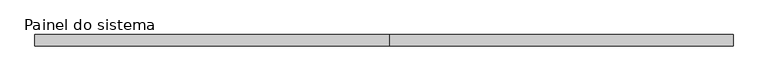
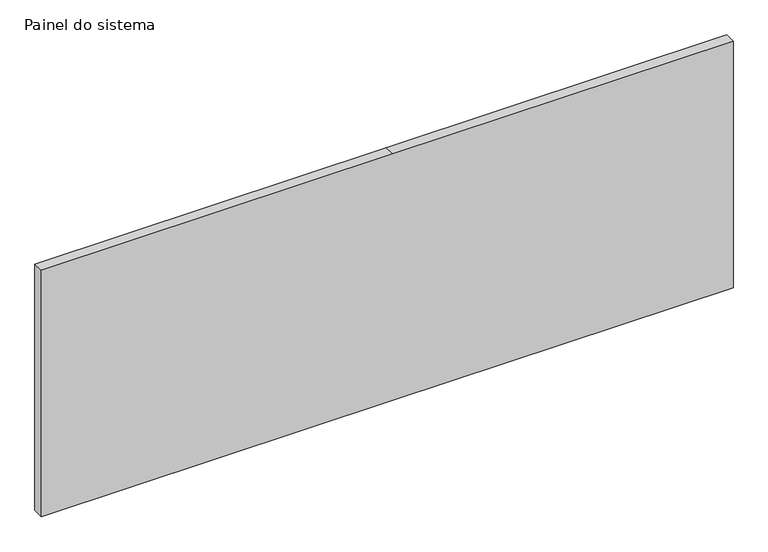
"""IFC4 building model written with IfcOpenShell, lengths in millimetres: plate geometry, Painel do sistema : Envidraçado."""

import ifcopenshell
import ifcopenshell.guid

model = None  # the IFC model being written
_history = None  # IfcOwnerHistory: only IFC2X3 demands one
_inside = {}  # id of a spatial element -> (the spatial element, [elements in it])
_under = {}  # id of a project, library or spatial element -> (it, [spatial elements below it])
_declared = {}  # id of a project -> (the project, [libraries it declares])
_typed = {}  # id of a type object -> (the type object, [elements of that type])
_made_of = {}  # id of a material, layer set ... -> (it, [elements and type objects made of it])


def new_model(schema):
    """Start an empty IFC model of exactly this schema.

    Asked for "IFC4X3", IfcOpenShell would pick the latest addendum, in which some entities
    have other attributes; the version numbers below select the first issue.
    IFC2X3 requires an IfcOwnerHistory on every rooted entity: one is made here for all.
    """
    global model, _history
    if schema == "IFC4X3":
        model = ifcopenshell.file(schema_version=(4, 3, 0, 0))
    else:
        model = ifcopenshell.file(schema=schema)
    _inside.clear()
    _under.clear()
    _declared.clear()
    _typed.clear()
    _made_of.clear()
    _history = None
    if model.schema == "IFC2X3":
        org = make("IfcOrganization", Name="unknown")
        user = make(
            "IfcPersonAndOrganization",
            ThePerson=make("IfcPerson", FamilyName="unknown"),
            TheOrganization=org,
        )
        app = make(
            "IfcApplication",
            ApplicationDeveloper=org,
            Version="unknown",
            ApplicationFullName="unknown",
            ApplicationIdentifier="unknown",
        )
        _history = make(
            "IfcOwnerHistory",
            OwningUser=user,
            OwningApplication=app,
            ChangeAction="ADDED",
            CreationDate=0,
        )
    return model


def make(cls, **values):
    """One entity of the class cls with the attributes given. An attribute that is None is left unset."""
    return model.create_entity(
        cls, **{name: value for name, value in values.items() if value is not None}
    )


def rooted(cls, **values):
    """An entity with a GlobalId (a new one), such as an element, a storey or a relation."""
    return make(cls, GlobalId=ifcopenshell.guid.new(), OwnerHistory=_history, **values)


def si_unit(unit_type, name, prefix=None):
    """IfcSIUnit, for example si_unit("LENGTHUNIT", "METRE", prefix="MILLI")."""
    return make("IfcSIUnit", UnitType=unit_type, Prefix=prefix, Name=name)


def assignment(units):
    """IfcUnitAssignment: the units of a project."""
    return None if units is None else make("IfcUnitAssignment", Units=units)


def point(xyz):
    """IfcCartesianPoint."""
    return None if xyz is None else make("IfcCartesianPoint", Coordinates=xyz)


def direction(xyz):
    """IfcDirection."""
    return None if xyz is None else make("IfcDirection", DirectionRatios=xyz)


def frame(location, z_axis=None, x_axis=None):
    """IfcAxis2Placement3D, a coordinate frame: its origin and axes. An axis left out is left unset."""
    return make(
        "IfcAxis2Placement3D",
        Location=point(location),
        Axis=direction(z_axis),
        RefDirection=direction(x_axis),
    )


def origin():
    """The frame at (0, 0, 0) with its axes left unset."""
    return frame((0.0, 0.0, 0.0))


def place(relative_to, where):
    """IfcLocalPlacement: puts the frame where relative to a parent placement (None: the world)."""
    return make(
        "IfcLocalPlacement", PlacementRelTo=relative_to, RelativePlacement=where
    )


def context(
    kind, dimensions, precision=None, world=None, true_north=None, identifier=None
):
    """IfcGeometricRepresentationContext, for example the 3D "Model" context."""
    return make(
        "IfcGeometricRepresentationContext",
        ContextIdentifier=identifier,
        ContextType=kind,
        CoordinateSpaceDimension=dimensions,
        Precision=precision,
        WorldCoordinateSystem=world,
        TrueNorth=true_north,
    )


def project(units=None, contexts=None):
    """IfcProject with its units and contexts."""
    return rooted(
        "IfcProject",
        Name="project",
        RepresentationContexts=contexts,
        UnitsInContext=assignment(units),
    )


def spatial(cls, under=None, at=None, **own):
    """A site, building, storey or space (cls), placed at a placement, below another one or the project."""
    s = rooted(cls, ObjectPlacement=at, **own)
    if under is not None:
        _under.setdefault(under.id(), (under, []))[1].append(s)
    return s


def polyline(points):
    """IfcPolyline through the points."""
    return make("IfcPolyline", Points=[point(p) for p in points])


def outline(outer, holes=None, kind="AREA"):
    """IfcArbitraryClosedProfileDef: a profile drawn as a closed curve; with holes, ...WithVoids."""
    if holes is None:
        return make("IfcArbitraryClosedProfileDef", ProfileType=kind, OuterCurve=outer)
    return make(
        "IfcArbitraryProfileDefWithVoids",
        ProfileType=kind,
        OuterCurve=outer,
        InnerCurves=holes,
    )


def extrude(swept, where, along, depth):
    """IfcExtrudedAreaSolid: the profile swept, set in the frame where, extruded along a direction by depth."""
    return make(
        "IfcExtrudedAreaSolid",
        SweptArea=swept,
        Position=where,
        ExtrudedDirection=direction(along),
        Depth=depth,
    )


def shape(context_of_items, identifier, shape_type, items):
    """IfcShapeRepresentation: the items that make up one representation, for example the "Body"."""
    return make(
        "IfcShapeRepresentation",
        ContextOfItems=context_of_items,
        RepresentationIdentifier=identifier,
        RepresentationType=shape_type,
        Items=items,
    )


def source(mapping_origin, context_of_items, identifier, shape_type, items):
    """IfcRepresentationMap: a shape defined once, which mapped items show again and again."""
    return make(
        "IfcRepresentationMap",
        MappingOrigin=mapping_origin,
        MappedRepresentation=shape(context_of_items, identifier, shape_type, items),
    )


def transform(
    local_origin,
    x_axis=None,
    y_axis=None,
    z_axis=None,
    scale=None,
    scale2=None,
    scale3=None,
    uniform=True,
):
    """IfcCartesianTransformationOperator3D, or its non-uniform kind. x_axis, y_axis, z_axis: its Axis1, 2, 3."""
    if uniform:
        return make(
            "IfcCartesianTransformationOperator3D",
            Axis1=direction(x_axis),
            Axis2=direction(y_axis),
            LocalOrigin=point(local_origin),
            Scale=scale,
            Axis3=direction(z_axis),
        )
    return make(
        "IfcCartesianTransformationOperator3DnonUniform",
        Axis1=direction(x_axis),
        Axis2=direction(y_axis),
        LocalOrigin=point(local_origin),
        Scale=scale,
        Axis3=direction(z_axis),
        Scale2=scale2,
        Scale3=scale3,
    )


def mapped(mapping_source, mapping_target):
    """IfcMappedItem: shows the shape of a source again, moved by a transform."""
    return make(
        "IfcMappedItem", MappingSource=mapping_source, MappingTarget=mapping_target
    )


def made_of(thing, what):
    """Note that an element or type object is made of a material, layer set ...; save() writes the relation."""
    if what is not None:
        _made_of.setdefault(what.id(), (what, []))[1].append(thing)
    return thing


def element(
    cls,
    number,
    at=None,
    inside=None,
    cuts=None,
    type_object=None,
    material=None,
    context=None,
    identifier="Body",
    shape_type=None,
    held_by="IfcProductDefinitionShape",
    body=None,
    shapes=None,
    **own,
):
    """One element of the class cls, such as IfcWall. Its Tag is "e" and its number.

    at: its placement. inside: the storey or other place that contains it. cuts: it is an
    opening in that element (IfcRelVoidsElement). A single representation is given by context,
    identifier, shape_type and body (its items); several are given by shapes. held_by: the class
    of the entity that holds the representations. save() writes the other relations.
    """
    e = rooted(cls, Tag="e%d" % number, ObjectPlacement=at, **own)
    if body is not None:
        shapes = [shape(context, identifier, shape_type, body)]
    if shapes is not None:
        e.Representation = make(held_by, Representations=shapes)
    if inside is not None:
        _inside.setdefault(inside.id(), (inside, []))[1].append(e)
    if cuts is not None:
        rooted(
            "IfcRelVoidsElement", RelatingBuildingElement=cuts, RelatedOpeningElement=e
        )
    if type_object is not None:
        _typed.setdefault(type_object.id(), (type_object, []))[1].append(e)
    return made_of(e, material)


def aggregate(whole, parts):
    """IfcRelAggregates: a whole, such as a stair, and the parts it consists of."""
    return rooted("IfcRelAggregates", RelatingObject=whole, RelatedObjects=parts)


def save(model, path):
    """Write the relations noted so far, then the file.

    IfcRelAggregates (storeys below a building ...), IfcRelContainedInSpatialStructure (elements
    in a storey), IfcRelDefinesByType, IfcRelAssociatesMaterial and IfcRelDeclares: one each for
    every whole, place, type object, material and project.
    """
    for whole, parts in _under.values():
        aggregate(whole, parts)
    for where, things in _inside.values():
        rooted(
            "IfcRelContainedInSpatialStructure",
            RelatedElements=things,
            RelatingStructure=where,
        )
    for kind, things in _typed.values():
        rooted("IfcRelDefinesByType", RelatedObjects=things, RelatingType=kind)
    for what, things in _made_of.values():
        rooted("IfcRelAssociatesMaterial", RelatedObjects=things, RelatingMaterial=what)
    for by, libraries in _declared.values():
        rooted("IfcRelDeclares", RelatingContext=by, RelatedDefinitions=libraries)
    model.write(path)


def painel_do_sistema_e8bc62b3(model_context):
    return source(origin(), model_context, "Body", "SweptSolid", [
        extrude(outline(polyline([(0.0, -783.4833334), (0.0, 12.4999998), (0.0, 783.4833334), (590.0, 783.4833334), (590.0, 12.4999998), (590.0, -783.4833334), (0.0, -783.4833334)])), frame((0.0, -49.5, 0.0), z_axis=(0.0, 1.0, 0.0), x_axis=(0.0, 0.0, 1.0)), (0.0, 0.0, 1.0), 25.0),
    ])


if __name__ == "__main__":
    model = new_model("IFC4")
    model_context = context("Model", 3, world=origin())
    ifc_project = project(units=[si_unit("LENGTHUNIT", "METRE", prefix="MILLI")], contexts=[model_context])
    site = spatial("IfcSite", under=ifc_project)
    building = spatial("IfcBuilding", under=site)
    placement = place(None, origin())
    painel_do_sistema_shape = painel_do_sistema_e8bc62b3(model_context)
    element("IfcPlate", 1, ObjectType="Painel do sistema : Envidraçado", at=placement, inside=building, context=model_context, shape_type="MappedRepresentation", body=[
        mapped(painel_do_sistema_shape, transform((0.0, 0.0, 0.0), x_axis=(1.0, 0.0, 0.0), y_axis=(0.0, 1.0, 0.0), z_axis=(0.0, 0.0, 1.0))),
    ])
    save(model, "model.ifc")

# Revit data of these elements
# Type "Painel do sistema : Envidraçado"
#   Construction Type Id = "GSP4R"
#   Analytic Construction = "Vidraça única Pilkington 1/8 pol"
#   Visual Light Transmittance = 0.9
#   Solar Heat Gain Coefficient = 0.86
#   Heat Transfer Coefficient (U) = 6.7069 W/(m²·K)
# Element 1 (IfcPlate, "Painel do sistema : Envidraçado")
#   Materials on its faces: ".VIDRO GENÉRICO"
# Materials
#   ".VIDRO GENÉRICO": class ".CC_VIDRO", colour RGB 0 128 192, transparency 0.9, Description = "Vidro comum", Cost = 0
